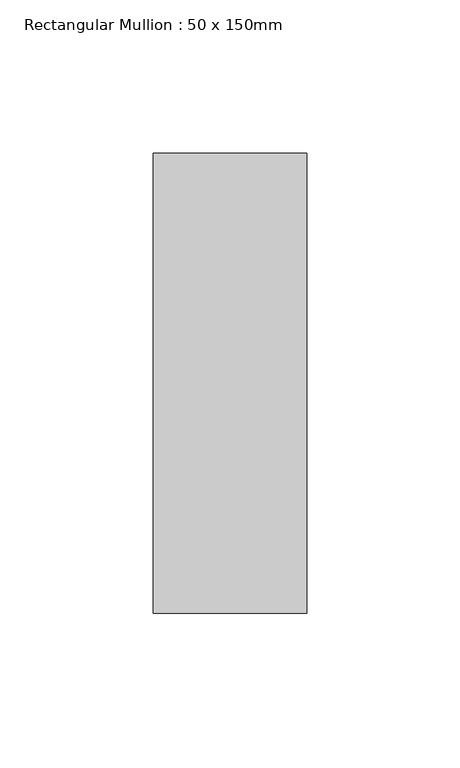
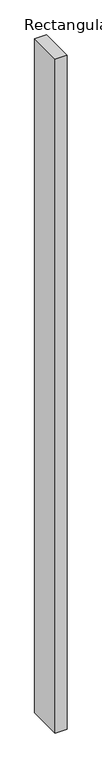
"""IFC4 building model written with IfcOpenShell, lengths in millimetres: member geometry, Rectangular Mullion : 50 x 150mm."""

from ifc_helpers import new_model, si_unit, frame, origin, place, context, project, spatial, polyline, outline, extrude, source, transform, mapped, element, save


def rectangular_mullion_50_x_150mm_68c91185(model_context):
    return source(origin(), model_context, "Body", "SweptSolid", [
        extrude(outline(polyline([(0.0, 75.0), (0.0, -75.0), (-50.0, -75.0), (-50.0, 75.0), (0.0, 75.0)])), frame((0.0, 0.0, -3000.0), z_axis=(0.0, 0.0, 1.0), x_axis=(1.0, 0.0, 0.0)), (0.0, 0.0, 1.0), 3000.0),
    ])


if __name__ == "__main__":
    model = new_model("IFC4")
    model_context = context("Model", 3, world=origin())
    ifc_project = project(units=[si_unit("LENGTHUNIT", "METRE", prefix="MILLI")], contexts=[model_context])
    site = spatial("IfcSite", under=ifc_project)
    building = spatial("IfcBuilding", under=site)
    placement = place(None, origin())
    rectangular_mullion_50_x_150mm_shape = rectangular_mullion_50_x_150mm_68c91185(model_context)
    element("IfcMember", 1, ObjectType="Rectangular Mullion : 50 x 150mm", at=placement, inside=building, context=model_context, shape_type="MappedRepresentation", body=[
        mapped(rectangular_mullion_50_x_150mm_shape, transform((0.0, 0.0, 0.0), x_axis=(1.0, 0.0, 0.0), y_axis=(0.0, 1.0, 0.0), z_axis=(0.0, 0.0, 1.0))),
    ])
    save(model, "model.ifc")

# Revit data of these elements
# Type "Rectangular Mullion : 50 x 150mm"
#   built-in parameter 1007304 = 0.492126 (stored number, unit not read)
#   built-in parameter 1007301 = 0.082021 (stored number, unit not read)
#   built-in parameter 1007300 = 0.082021 (stored number, unit not read)
# Element 1 (IfcMember, "Rectangular Mullion : 50 x 150mm")
#   Materials on its faces: "Metal - Aluminium"
# Materials
#   "Metal - Aluminium": class "Metal", colour RGB 247 247 247, transparency 0
